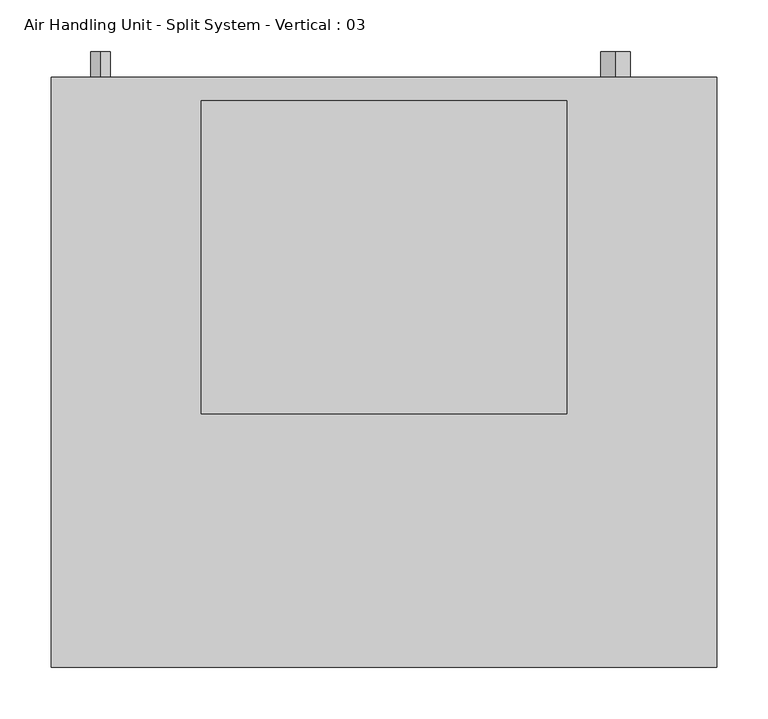
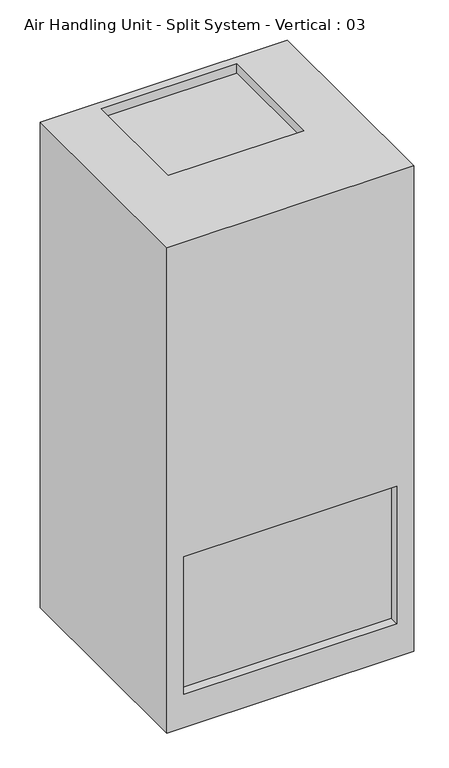
"""IFC4 building model written with IfcOpenShell, lengths in millimetres: proxy geometry, Air Handling Unit - Split System - Vertical : 03."""

from ifc_helpers import new_model, si_unit, point, frame, frame_2d, origin, place, context, project, spatial, circle_curve, trimmed, segment, composite_curve, outline, extrude, faceted_brep, source, transform, mapped, element, save


def air_handling_unit_split_system_vertical_03_658e3e83(model_context):
    return source(origin(), model_context, "Body", "SolidModel", [
        extrude(outline(composite_curve([segment(trimmed(circle_curve(frame_2d((132.55625, -275.828125)), 9.525), [point((142.08125, -275.828125))], [point((123.03125, -275.828125))], False, "CARTESIAN"), True, "CONTINUOUS"), segment(trimmed(circle_curve(frame_2d((132.55625, -275.828125)), 9.525), [point((123.03125, -275.828125))], [point((142.08125, -275.828125))], False, "CARTESIAN"), True, "CONTINUOUS")], self_intersect=False)), frame((0.0, 287.0398438, 0.0), z_axis=(0.0, 1.0, 0.0), x_axis=(0.0, 0.0, 1.0)), (0.0, 0.0, 1.0), 25.4),
        extrude(outline(composite_curve([segment(trimmed(circle_curve(frame_2d((394.096875, 225.425)), 4.7625), [point((398.859375, 225.425))], [point((389.334375, 225.425))], False, "CARTESIAN"), True, "CONTINUOUS"), segment(trimmed(circle_curve(frame_2d((394.096875, 225.425)), 4.7625), [point((389.334375, 225.425))], [point((398.859375, 225.425))], False, "CARTESIAN"), True, "CONTINUOUS")], self_intersect=False)), frame((0.0, 287.0398438, 0.0), z_axis=(0.0, 1.0, 0.0), x_axis=(0.0, 0.0, 1.0)), (0.0, 0.0, 1.0), 25.4),
        extrude(outline(composite_curve([segment(trimmed(circle_curve(frame_2d((465.534375, 225.425)), 14.2875), [point((479.821875, 225.425))], [point((451.246875, 225.425))], False, "CARTESIAN"), True, "CONTINUOUS"), segment(trimmed(circle_curve(frame_2d((465.534375, 225.425)), 14.2875), [point((451.246875, 225.425))], [point((479.821875, 225.425))], False, "CARTESIAN"), True, "CONTINUOUS")], self_intersect=False)), frame((0.0, 287.0398438, 0.0), z_axis=(0.0, 1.0, 0.0), x_axis=(0.0, 0.0, 1.0)), (0.0, 0.0, 1.0), 25.4),
        faceted_brep([(323.85, 287.0398438, 1346.2), (-323.85, 287.0398438, 1346.2), (-323.85, -287.0398438, 1346.2), (323.85, -287.0398438, 1346.2), (177.8, 264.2195313, 1346.2), (177.8, -40.5804687, 1346.2), (-177.8, -40.5804687, 1346.2), (-177.8, 264.2195313, 1346.2), (323.85, 287.0398438, 0.0), (323.85, -287.0398438, 0.0), (-323.85, -287.0398438, 0.0), (-323.85, 287.0398438, 0.0), (279.4, -287.0398438, 472.8765625), (279.4, -287.0398438, 91.8765625), (-279.4, -287.0398438, 91.8765625), (-279.4, -287.0398438, 472.8765625), (177.8, 264.2195313, 1320.8), (-177.8, 264.2195313, 1320.8), (-177.8, -40.5804687, 1320.8), (177.8, -40.5804687, 1320.8), (279.4, -261.6398438, 472.8765625), (-279.4, -261.6398438, 472.8765625), (-279.4, -261.6398438, 91.8765625), (279.4, -261.6398438, 91.8765625)], [[[0, 1, 2, 3], [4, 5, 6, 7]], [[8, 9, 10, 11]], [[1, 0, 8, 11]], [[2, 1, 11, 10]], [[3, 2, 10, 9], [12, 13, 14, 15]], [[0, 3, 9, 8]], [[16, 17, 18, 19]], [[16, 19, 5, 4]], [[19, 18, 6, 5]], [[18, 17, 7, 6]], [[17, 16, 4, 7]], [[20, 21, 22, 23]], [[20, 23, 13, 12]], [[23, 22, 14, 13]], [[22, 21, 15, 14]], [[21, 20, 12, 15]]]),
    ])


if __name__ == "__main__":
    model = new_model("IFC4")
    model_context = context("Model", 3, world=origin())
    ifc_project = project(units=[si_unit("LENGTHUNIT", "METRE", prefix="MILLI")], contexts=[model_context])
    site = spatial("IfcSite", under=ifc_project)
    building = spatial("IfcBuilding", under=site)
    placement = place(None, origin())
    air_handling_unit_split_system_vertical_03_shape = air_handling_unit_split_system_vertical_03_658e3e83(model_context)
    element("IfcBuildingElementProxy", 1, Name="Air Handling Unit - Split System - Vertical : 03", ObjectType="Air Handling Unit - Split System - Vertical : 03", at=placement, inside=building, context=model_context, shape_type="MappedRepresentation", body=[
        mapped(air_handling_unit_split_system_vertical_03_shape, transform((0.0, 0.0, 0.0), x_axis=(1.0, 0.0, 0.0), y_axis=(0.0, 1.0, 0.0), z_axis=(0.0, 0.0, 1.0))),
    ])
    save(model, "model.ifc")

# Revit data of these elements
# Project information
#   Project Issue Date = "Issue Date"
#   Project Status = "Project Status"
#   Client Name = "Owner"
#   Project Address = "Enter address here"
#   Project Name = "Project Name"
#   Project Number = "Project Number"
# Type "Air Handling Unit - Split System - Vertical : 03"
#   PartShape = "Rectangular Duct"
#   Model = "03"
#   Voltage = 208 V
#   UnitWidth = 2' - 1 1/2"
#   UnitHeight = 4' - 5"
#   UnitDepth = 1' - 10 77/128"
#   Width1 = 1' - 2"
#   SupplyOpeningOffset = 0' - 0 115/128"
#   Outlet Radius = 9/16"
#   Outlet Diameter = 1 1/8"
#   Inlet Radius = 3/16"
#   Inlet Diameter = 3/8"
#   Height1 = 1' - 0"
#   SupplyConnectorOffset = 0' - 6"
#   Width2 = 1' - 10"
#   Height2 = 1' - 3"
#   ReturnConnectorOffset = 0' - 7 1/2"
#   ReturnAirOffset = 0' - 3 79/128"
#   Half UnitWidth = 1' - 0 3/4"
#   Drain Flow [instance default] = 0 GPM
#   C3 Offset 1 = 1' - 6 21/64"
#   Apparent Load = 10816 VA
#   External Static Pressure [instance default] = 0.50 in-wg
#   Air Flow [instance default] = 1170 CFM
#   Number of Poles = 3
#   Load Classification = Cooling
#   Default Elevation = 0
#   Assembly Code = ""
